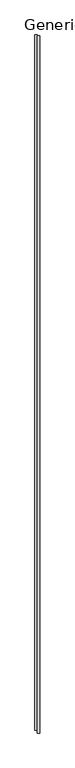
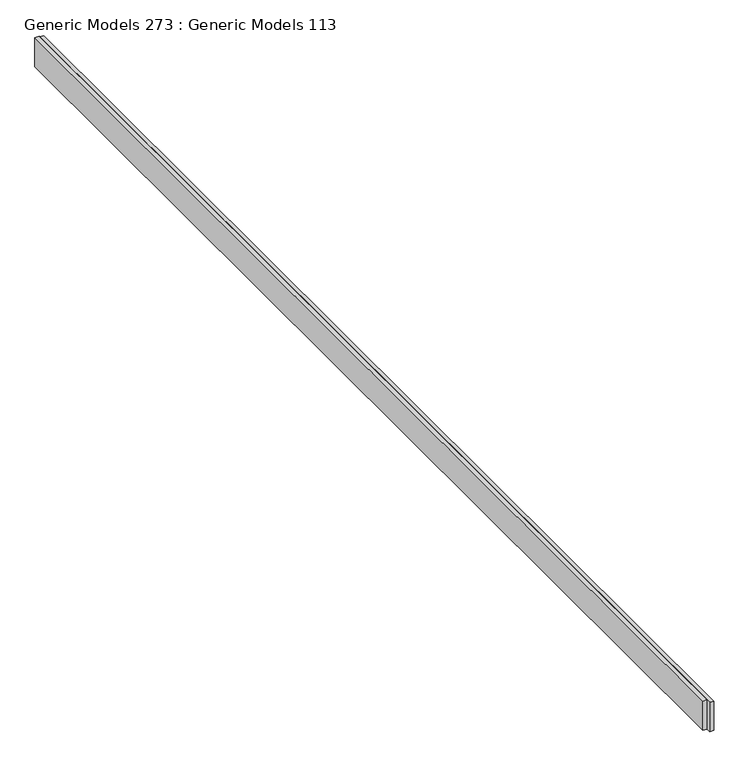
"""IFC4 building model written with IfcOpenShell, lengths in millimetres: proxy geometry, Generic Models 273 : Generic Models 113."""

from ifc_helpers import new_model, si_unit, frame, origin, place, context, project, spatial, polyline, outline, extrude, source, transform, mapped, element, save


def generic_models_273_generic_models_113_8922fb19(model_context):
    return source(origin(), model_context, "Body", "SweptSolid", [
        extrude(outline(polyline([(32129.4210525, 39325.7063104), (32167.5210525, 39325.7063104), (32167.5210525, 28631.9337847), (32129.4210525, 28631.9337847), (32129.4210525, 39325.7063104)])), frame((0.0, 0.0, 266084.05), z_axis=(0.0, 0.0, 1.0), x_axis=(1.0, 0.0, 0.0)), (0.0, 0.0, 1.0), 285.75),
        extrude(outline(polyline([(32091.3210525, 39335.730832), (32129.4210525, 39335.730832), (32129.4210525, 28673.6427519), (32091.3210525, 28673.6427519), (32091.3210525, 39335.730832)])), frame((0.0, 0.0, 266084.05), z_axis=(0.0, 0.0, 1.0), x_axis=(1.0, 0.0, 0.0)), (0.0, 0.0, 1.0), 285.75),
    ])


if __name__ == "__main__":
    model = new_model("IFC4")
    model_context = context("Model", 3, world=origin())
    ifc_project = project(units=[si_unit("LENGTHUNIT", "METRE", prefix="MILLI")], contexts=[model_context])
    site = spatial("IfcSite", under=ifc_project)
    building = spatial("IfcBuilding", under=site)
    placement = place(None, origin())
    generic_models_273_generic_models_113_shape = generic_models_273_generic_models_113_8922fb19(model_context)
    element("IfcBuildingElementProxy", 1, Name="Generic Models 273 : Generic Models 113", ObjectType="Generic Models 273 : Generic Models 113", at=placement, inside=building, context=model_context, shape_type="MappedRepresentation", body=[
        mapped(generic_models_273_generic_models_113_shape, transform((0.0, 0.0, 0.0), x_axis=(1.0, 0.0, 0.0), y_axis=(0.0, 1.0, 0.0), z_axis=(0.0, 0.0, 1.0))),
    ])
    save(model, "model.ifc")

# Revit data of these elements
# Element 1 (IfcBuildingElementProxy, "Generic Models 273 : Generic Models 113")
#   Materials on its faces: "(2) TREATED 2X12's"
# Materials
#   "(2) TREATED 2X12's": class "Wood", colour RGB 144 113 62, transparency 0, Description = "Pinus Echinata", Cost = 0
